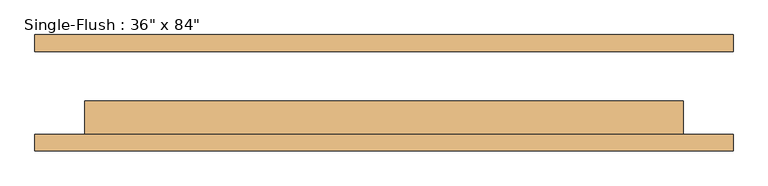
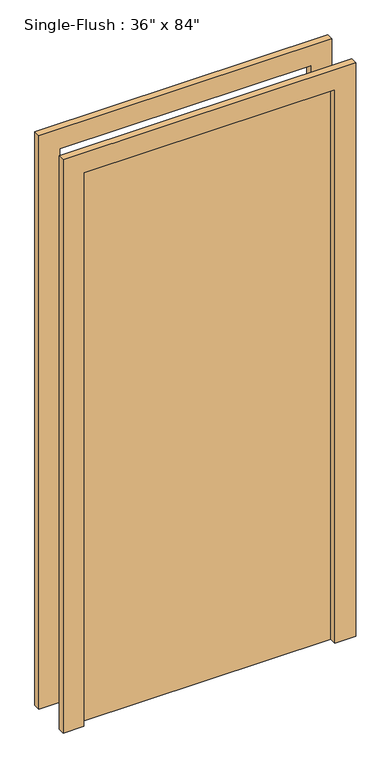
"""IFC4 building model written with IfcOpenShell, lengths in millimetres: door geometry."""

from ifc_helpers import new_model, si_unit, frame, origin, origin_with_axes, place, context, project, spatial, polyline, outline, extrude, source, transform, mapped, element, save


def door_a3eb833a(model_context):
    return source(origin(), model_context, "Body", "SweptSolid", [
        extrude(outline(polyline([(2209.8, -533.4), (0.0, -533.4), (0.0, -457.2), (2133.6, -457.2), (2133.6, 457.2), (0.0, 457.2), (0.0, 533.4), (2209.8, 533.4), (2209.8, -533.4)])), frame((0.0, -88.9, 0.0), z_axis=(0.0, 1.0, 0.0), x_axis=(0.0, 0.0, 1.0)), (0.0, 0.0, 1.0), 25.4),
        extrude(outline(polyline([(2209.8, 533.4), (2209.8, -533.4), (0.0, -533.4), (0.0, -457.2), (2133.6, -457.2), (2133.6, 457.2), (0.0, 457.2), (0.0, 533.4), (2209.8, 533.4)])), frame((0.0, 63.5, 0.0), z_axis=(0.0, 1.0, 0.0), x_axis=(0.0, 0.0, 1.0)), (0.0, 0.0, 1.0), 25.4),
        extrude(outline(polyline([(457.2, -12.7), (457.2, -63.5), (-457.2, -63.5), (-457.2, -12.7), (457.2, -12.7)])), origin_with_axes(), (0.0, 0.0, 1.0), 2133.6),
    ])


if __name__ == "__main__":
    model = new_model("IFC4")
    model_context = context("Model", 3, world=origin())
    ifc_project = project(units=[si_unit("LENGTHUNIT", "METRE", prefix="MILLI")], contexts=[model_context])
    site = spatial("IfcSite", under=ifc_project)
    building = spatial("IfcBuilding", under=site)
    placement = place(None, origin())
    door_shape = door_a3eb833a(model_context)
    element("IfcDoor", 1, ObjectType="Single-Flush : 36\" x 84\"", at=placement, inside=building, context=model_context, shape_type="MappedRepresentation", body=[
        mapped(door_shape, transform((0.0, 0.0, 0.0), x_axis=(1.0, 0.0, 0.0), y_axis=(0.0, 1.0, 0.0), z_axis=(0.0, 0.0, 1.0))),
    ])
    save(model, "model.ifc")

# Revit data of these elements
# Type "Single-Flush : 36\" x 84\""
#   Type Mark = "8"
#   Construction Type Id = "MDOOR"
#   Assembly Code = "C1020"
#   Analytic Construction = "Metal"
#   Thickness = 0' - 2"
#   Heat Transfer Coefficient (U) = 0.651978 BTU/(h·ft²·°F)
#   Height = 7' - 0"
#   Trim Projection Ext = 0' - 1"
#   Trim Projection Int = 0' - 1"
#   Trim Width = 0' - 3"
#   Width = 3' - 0"
#   Define Thermal Properties by = 1
#   Define Thermal Properties by = 1
#   Door Material = Door - Panel
#   Frame Material = Door - Frame
#   Visual Light Transmittance = 0
#   Solar Heat Gain Coefficient = 0
#   Function = (empty or 0)
#   Wall Closure = (empty or 0)
# Element 1 (IfcDoor, "Single-Flush : 36\" x 84\"")
#   Materials on its faces: "Door - Frame", "Door - Panel"
# Materials
#   "Door - Panel": class "Wood", colour RGB 210 159 95, transparency 0
#   "Door - Frame": class "Miscellaneous", colour RGB 118 70 51, transparency 0
